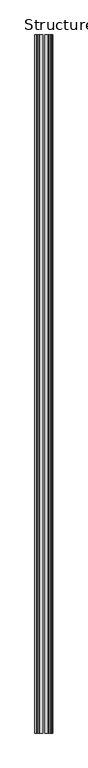
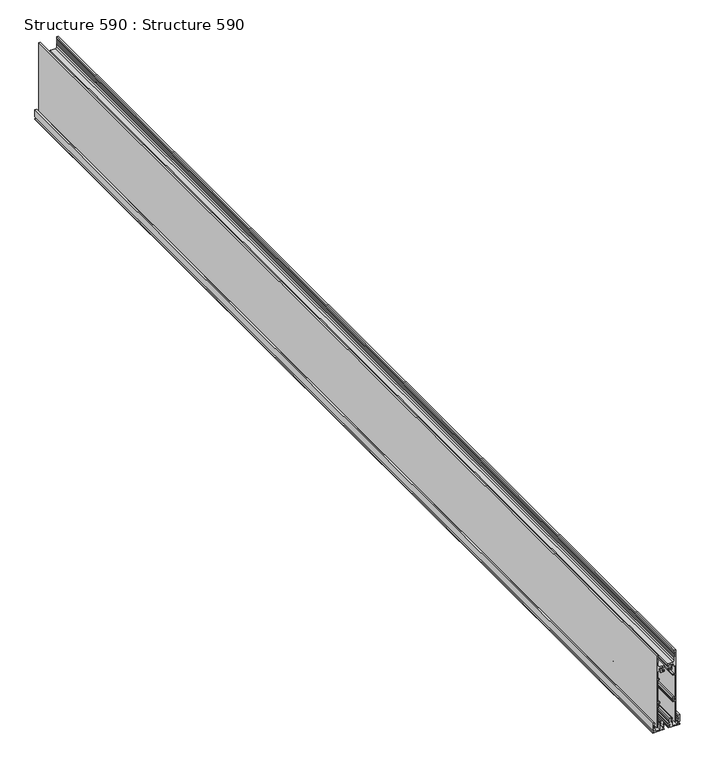
"""IFC4 building model written with IfcOpenShell, lengths in millimetres: proxy geometry, Structure 590 : Structure 590."""

from ifc_helpers import new_model, si_unit, frame, origin, place, context, project, spatial, polyline, outline, extrude, source, transform, mapped, element, save


def structure_590_structure_590_65a09181(model_context):
    return source(origin(), model_context, "Body", "SweptSolid", [
        extrude(outline(polyline([(37496.4365618, 7606.8679227), (37495.366697, 7605.8277084), (37493.1734209, 7605.8277084), (37493.1734209, 7606.8978655), (37494.7782571, 7606.8978655), (37494.7782571, 7608.235562), (37486.7569596, 7608.235562), (37486.7569596, 7606.8978655), (37488.3589123, 7606.8978655), (37488.3589123, 7605.8277084), (37485.0752597, 7605.8277084), (37483.4739937, 7604.9715826), (37479.1043438, 7604.9715826), (37479.1043438, 7595.9287546), (37488.3579135, 7595.9287546), (37488.3579135, 7594.8585974), (37486.7540761, 7594.8585974), (37486.7540761, 7593.520901), (37494.7782571, 7593.520901), (37494.7782571, 7594.8585974), (37493.1734209, 7594.8585974), (37493.1734209, 7595.9287546), (37495.366697, 7595.9287546), (37496.436721, 7594.8587306), (37496.436721, 7593.7884403), (37495.5512233, 7591.7164162), (37493.0931791, 7590.4441991), (37490.017243, 7590.4441991), (37490.017243, 7591.5143563), (37486.4063615, 7591.5143563), (37486.4063615, 7588.8385466), (37484.5340526, 7588.8385466), (37484.5340526, 7589.6419937), (37483.2789107, 7589.6419937), (37484.4508456, 7591.1523679), (37484.4508456, 7592.2741958), (37480.1257911, 7592.2741958), (37479.7006783, 7593.0033391), (37479.2397502, 7592.248166), (37479.2397502, 7590.8512242), (37480.6168771, 7590.8512242), (37480.6168771, 7589.3613824), (37479.8959721, 7588.7994279), (37477.446, 7588.6064565), (37477.446, 7590.7198342), (37478.4679055, 7590.7198342), (37478.4679055, 7592.2741958), (37477.446, 7592.2741958), (37477.446, 7610.108337), (37478.8903656, 7610.108337), (37478.8903656, 7606.6303263), (37484.2874925, 7606.6303263), (37483.0336251, 7608.7837666), (37483.0336251, 7610.108337), (37496.4365618, 7610.108337), (37496.4365618, 7606.8679227)])), frame((0.0, -3747.9491938, 0.0), z_axis=(0.0, 1.0, 0.0), x_axis=(0.0, 0.0, 1.0)), (0.0, 0.0, 1.0), 2000.0),
        extrude(outline(polyline([(37483.0336251, 7559.1546644), (37483.0336251, 7560.4792348), (37484.2874925, 7562.6326752), (37478.8903656, 7562.6326752), (37478.8903656, 7559.1546644), (37477.446, 7559.1546644), (37477.446, 7576.9888056), (37478.4679055, 7576.9888056), (37478.4679055, 7578.5431673), (37477.446, 7578.5431673), (37477.446, 7580.6565449), (37479.8959721, 7580.4635736), (37480.6168771, 7579.9016191), (37480.6168771, 7578.4117772), (37479.2397502, 7578.4117772), (37479.2397502, 7577.0148355), (37479.7006783, 7576.2596623), (37480.1257911, 7576.9888056), (37484.4508456, 7576.9888056), (37484.4508456, 7578.1106336), (37483.2789107, 7579.6210078), (37484.5340526, 7579.6210078), (37484.5340526, 7580.4244548), (37486.4063615, 7580.4244548), (37486.4063615, 7577.7486452), (37490.017243, 7577.7486452), (37490.017243, 7578.8188023), (37493.0931791, 7578.8188023), (37495.5512233, 7577.5465852), (37496.436721, 7575.4745612), (37496.436721, 7574.4042708), (37495.366697, 7573.3342469), (37493.1734209, 7573.3342469), (37493.1734209, 7574.404404), (37494.7782571, 7574.404404), (37494.7782571, 7575.7421005), (37486.7540761, 7575.7421005), (37486.7540761, 7574.404404), (37488.3579135, 7574.404404), (37488.3579135, 7573.3342469), (37479.1043438, 7573.3342469), (37479.1043438, 7564.2914188), (37483.4739937, 7564.2914188), (37485.0752597, 7563.4352931), (37488.3589123, 7563.4352931), (37488.3589123, 7562.3651359), (37486.7569596, 7562.3651359), (37486.7569596, 7561.0274394), (37494.7782571, 7561.0274394), (37494.7782571, 7562.3651359), (37493.1734209, 7562.3651359), (37493.1734209, 7563.4352931), (37495.366697, 7563.4352931), (37496.4365618, 7562.3950788), (37496.4365618, 7559.1546644), (37483.0336251, 7559.1546644)])), frame((0.0, -3747.9491938, 0.0), z_axis=(0.0, 1.0, 0.0), x_axis=(0.0, 0.0, 1.0)), (0.0, 0.0, 1.0), 2000.0),
        extrude(outline(polyline([(37604.2015618, 7571.6095342), (37606.7094313, 7569.1016647), (37611.5111794, 7569.1016647), (37613.3758754, 7569.5762356), (37616.0506024, 7568.7736177), (37616.0506024, 7569.5762356), (37618.7253294, 7568.7736177), (37618.7253294, 7569.5762356), (37621.4000564, 7568.7736177), (37621.4000564, 7569.5762356), (37624.0747835, 7568.7736177), (37624.0747835, 7569.5762356), (37626.7495105, 7569.5762356), (37626.7495105, 7566.5797955), (37485.4971771, 7566.5797955), (37485.4971771, 7569.0946649), (37525.8320604, 7569.0946649), (37525.8320604, 7571.9840892), (37527.4903911, 7571.9840892), (37527.4903911, 7571.0209478), (37529.4164343, 7569.0949046), (37532.9735815, 7569.0949046), (37532.9735815, 7570.913932), (37531.2885035, 7570.913932), (37531.2885035, 7572.5191678), (37534.6319122, 7572.5191678), (37534.6319122, 7569.0946649), (37578.3369516, 7569.0946649), (37578.3369516, 7571.9840892), (37579.9952823, 7571.9840892), (37579.9952823, 7569.0946649), (37595.9502358, 7569.0946649), (37595.9502358, 7570.0103582), (37597.8865057, 7571.2830063), (37599.3688896, 7570.5326641), (37600.7763445, 7570.5326641), (37601.7660928, 7572.4667938), (37600.8580603, 7574.2374752), (37599.3688896, 7574.2374752), (37597.8866262, 7573.5415066), (37595.9502358, 7574.6594821), (37591.6838394, 7574.6594821), (37591.6838394, 7581.3479644), (37594.6795336, 7581.3479644), (37594.6795336, 7580.010268), (37593.3421701, 7580.010268), (37593.3421701, 7576.3182257), (37601.6873184, 7576.3182257), (37601.6873184, 7580.010268), (37600.3499549, 7580.010268), (37600.3499549, 7581.3479644), (37604.2015618, 7581.3479644), (37604.2015618, 7571.6095342)])), frame((0.0, -3747.9491938, 0.0), z_axis=(0.0, 1.0, 0.0), x_axis=(0.0, 0.0, 1.0)), (0.0, 0.0, 1.0), 2000.0),
        extrude(outline(polyline([(37600.3499549, 7587.915037), (37600.3499549, 7589.2527335), (37601.6873184, 7589.2527335), (37601.6873184, 7592.9447757), (37593.3421701, 7592.9447757), (37593.3421701, 7589.2527335), (37594.6795336, 7589.2527335), (37594.6795336, 7587.915037), (37591.6838394, 7587.915037), (37591.6838394, 7594.6035193), (37595.9502358, 7594.6035193), (37597.8866262, 7595.7214949), (37599.3688896, 7595.0255262), (37600.8580603, 7595.0255262), (37601.7660928, 7596.7962076), (37600.7763445, 7598.7303373), (37599.3688896, 7598.7303373), (37597.8865057, 7597.9799951), (37595.9502358, 7599.2526433), (37595.9502358, 7600.1683366), (37579.9952823, 7600.1683366), (37579.9952823, 7597.2789122), (37578.3369516, 7597.2789122), (37578.3369516, 7600.1683366), (37534.6319122, 7600.1683366), (37534.6319122, 7596.7438337), (37531.2885035, 7596.7438337), (37531.2885035, 7598.3490694), (37532.9735815, 7598.3490694), (37532.9735815, 7600.1680969), (37529.4164343, 7600.1680969), (37527.4903911, 7598.2420537), (37527.4903911, 7597.2789122), (37525.8320604, 7597.2789122), (37525.8320604, 7600.1683366), (37485.4971771, 7600.1683366), (37485.4971771, 7602.6832059), (37626.7495105, 7602.6832059), (37626.7495105, 7599.6867659), (37624.0747835, 7599.6867659), (37624.0747835, 7600.4893837), (37621.4000564, 7599.6867659), (37621.4000564, 7600.4893837), (37618.7253294, 7599.6867659), (37618.7253294, 7600.4893837), (37616.0506024, 7599.6867659), (37616.0506024, 7600.4893837), (37613.3758754, 7599.6867659), (37611.5111794, 7600.1613368), (37606.7094313, 7600.1613368), (37604.2015618, 7597.6534672), (37604.2015618, 7587.915037), (37600.3499549, 7587.915037)])), frame((0.0, -3747.9491938, 0.0), z_axis=(0.0, 1.0, 0.0), x_axis=(0.0, 0.0, 1.0)), (0.0, 0.0, 1.0), 2000.0),
    ])


if __name__ == "__main__":
    model = new_model("IFC4")
    model_context = context("Model", 3, world=origin())
    ifc_project = project(units=[si_unit("LENGTHUNIT", "METRE", prefix="MILLI")], contexts=[model_context])
    site = spatial("IfcSite", under=ifc_project)
    building = spatial("IfcBuilding", under=site)
    placement = place(None, origin())
    structure_590_structure_590_shape = structure_590_structure_590_65a09181(model_context)
    element("IfcBuildingElementProxy", 1, Name="Structure 590 : Structure 590", ObjectType="Structure 590 : Structure 590", at=placement, inside=building, context=model_context, shape_type="MappedRepresentation", body=[
        mapped(structure_590_structure_590_shape, transform((0.0, 0.0, 0.0), x_axis=(1.0, 0.0, 0.0), y_axis=(0.0, 1.0, 0.0), z_axis=(0.0, 0.0, 1.0))),
    ])
    save(model, "model.ifc")

# Revit data of these elements
# Type "Structure 590 : Structure 590"
#   NameOverride = "Structure"
# Element 1 (IfcBuildingElementProxy, "Structure 590 : Structure 590")
#   Materials on its faces: "FLEETWOOD SLIDING DOOR SERIES 3070 (SEE ELEVATIONS FOR OPERABILITY)"
# Materials
#   "FLEETWOOD SLIDING DOOR SERIES 3070 (SEE ELEVATIONS FOR OPERABILITY)": class "Unassigned", colour RGB 143 136 136, transparency 0, Cost = 0
